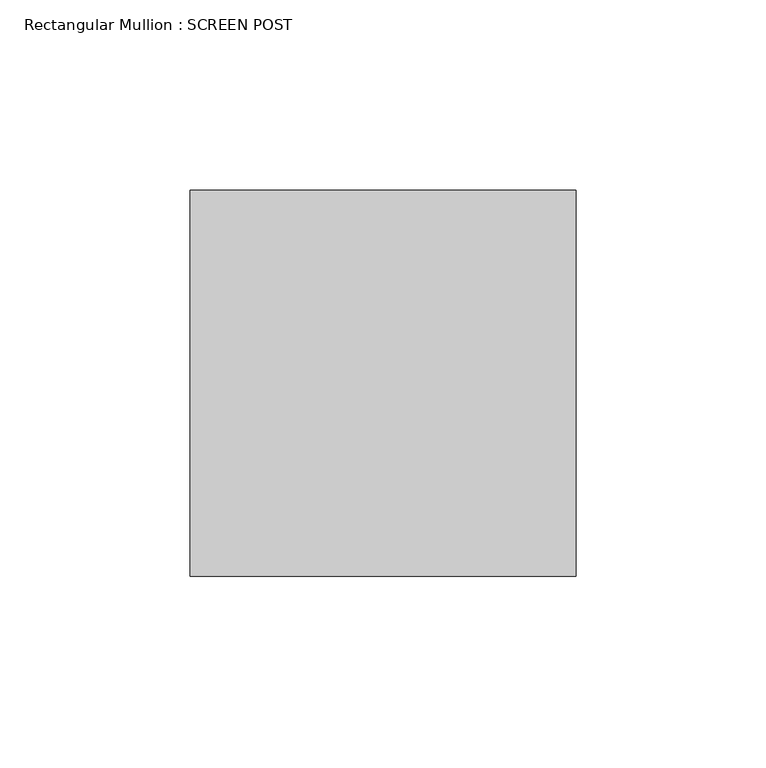
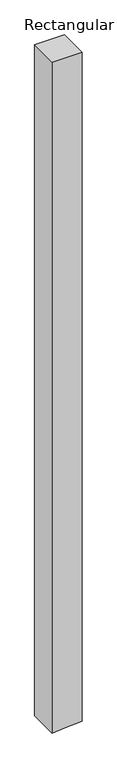
"""IFC4 building model written with IfcOpenShell, lengths in millimetres: member geometry, Rectangular Mullion : SCREEN POST."""

from ifc_helpers import new_model, si_unit, frame, origin, place, context, project, spatial, polyline, outline, extrude, source, transform, mapped, element, save


def rectangular_mullion_screen_post_311850e6(model_context):
    return source(origin(), model_context, "Body", "SweptSolid", [
        extrude(outline(polyline([(0.0, 50.8), (0.0, -50.8), (-2400.8656619, -50.8), (-2398.0824576, -6.3490391), (-2394.5041897, 50.8), (0.0, 50.8)])), frame((0.0, -50.8, 0.0), z_axis=(0.0, 1.0, 0.0), x_axis=(0.0, 0.0, 1.0)), (0.0, 0.0, 1.0), 101.6),
    ])


if __name__ == "__main__":
    model = new_model("IFC4")
    model_context = context("Model", 3, world=origin())
    ifc_project = project(units=[si_unit("LENGTHUNIT", "METRE", prefix="MILLI")], contexts=[model_context])
    site = spatial("IfcSite", under=ifc_project)
    building = spatial("IfcBuilding", under=site)
    placement = place(None, origin())
    rectangular_mullion_screen_post_shape = rectangular_mullion_screen_post_311850e6(model_context)
    element("IfcMember", 1, ObjectType="Rectangular Mullion : SCREEN POST", at=placement, inside=building, context=model_context, shape_type="MappedRepresentation", body=[
        mapped(rectangular_mullion_screen_post_shape, transform((0.0, 0.0, 0.0), x_axis=(1.0, 0.0, 0.0), y_axis=(0.0, 1.0, 0.0), z_axis=(0.0, 0.0, 1.0))),
    ])
    save(model, "model.ifc")

# Revit data of these elements
# Type "Rectangular Mullion : SCREEN POST"
#   built-in parameter 1007304 = 0.333333 (stored number, unit not read)
#   built-in parameter 1007301 = 0.166667 (stored number, unit not read)
#   built-in parameter 1007300 = 0.166667 (stored number, unit not read)
# Element 1 (IfcMember, "Rectangular Mullion : SCREEN POST")
#   Materials on its faces: "SCREEN PORCH FRAMING"
# Materials
#   "SCREEN PORCH FRAMING": class "Wood", colour RGB 164 134 123, transparency 0, Description = "Pinus Echinata", Cost = 0
